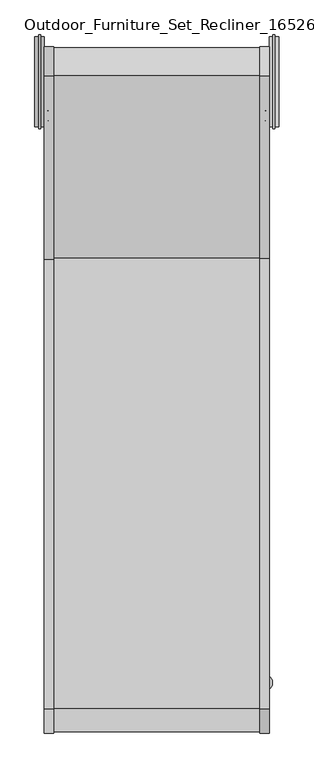
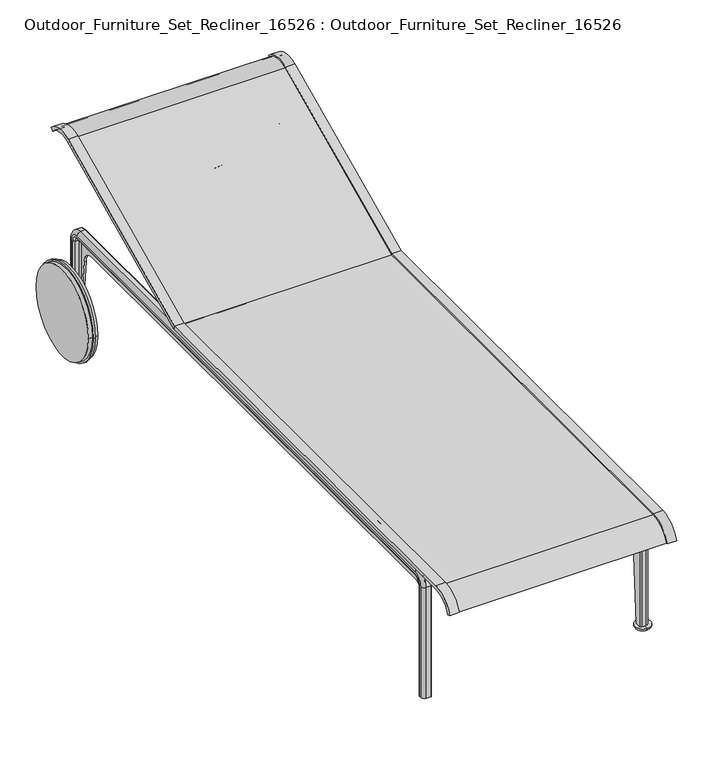
"""IFC4 building model written with IfcOpenShell, lengths in millimetres: furniture geometry, Outdoor_Furniture_Set_Recliner_16526 : Outdoor_Furniture_Set_Recliner_16526."""

from ifc_helpers import new_model, si_unit, point, frame, frame_2d, origin, place, context, project, spatial, polyline, circle_curve, ellipse_curve, trimmed, segment, composite_curve, outline, extrude, source, transform, mapped, element, save
from ifc_brep_helpers import plane_surface, cylinder_surface, revolved_surface, advanced_brep


def outdoor_furniture_set_recliner_16526_outdoor_furniture_set_cea44930(model_context):
    return source(origin(), model_context, "Body", "SolidModel", [
        advanced_brep(
        [(-276.0, -774.0474114, 267.1028811), (-276.0, -739.0647921, 301.0), (-276.0, 739.0647921, 301.0), (-276.0, 774.0474114, 267.1028811), (-276.0, 790.0, 100.0), (-276.0, 807.0, 100.0), (-276.0, 807.0, 320.0), (-276.0, 775.0, 352.0), (-276.0, -775.0, 352.0), (-276.0, -807.0, 320.0), (-276.0, -807.0, 10.0), (-276.0, -790.0, 10.0), (-281.0, 774.0474114, 267.1028811), (-281.0, 739.0647921, 301.0), (-281.0, -739.0647921, 301.0), (-281.0, -774.0474114, 267.1028811), (-281.0, -785.0, 90.583436), (-281.0, -785.0, 320.0), (-281.0, -775.0, 330.0), (-281.0, 775.0, 330.0), (-281.0, 785.0, 320.0), (-281.0, 785.0, 152.374848), (-286.0, 790.0, 100.0), (-286.0, -790.0, 10.0), (-295.0, 790.0, 100.0), (-300.0, 795.0, 100.0), (-300.0, 800.0, 100.0), (-290.0, 810.0, 100.0), (-279.0, 810.0, 100.0), (-290.0, 810.0, 320.0), (-279.0, 810.0, 320.0), (-295.0, 790.0, 320.0), (-286.0, 790.0, 320.0), (-290.0, 775.0, 355.0), (-279.0, 775.0, 355.0), (-295.0, 775.0, 335.0), (-286.0, 775.0, 335.0), (-290.0, -775.0, 355.0), (-279.0, -775.0, 355.0), (-295.0, -775.0, 335.0), (-286.0, -775.0, 335.0), (-290.0, -810.0, 320.0), (-279.0, -810.0, 320.0), (-295.0, -790.0, 320.0), (-286.0, -790.0, 320.0), (-279.0, -810.0, 10.0), (-290.0, -810.0, 10.0), (-300.0, -800.0, 10.0), (-300.0, -795.0, 10.0), (-295.0, -790.0, 10.0), (-300.0, 795.0, 320.0), (-300.0, 775.0, 340.0), (-300.0, -775.0, 340.0), (-300.0, -795.0, 320.0), (-300.0, -800.0, 320.0), (-300.0, -775.0, 345.0), (-300.0, 775.0, 345.0), (-300.0, 800.0, 320.0)],
        [
            (0, 1, circle_curve(frame((-276.0, -739.0647921, 266.0), z_axis=(-1.0, 0.0, 0.0), x_axis=(0.0, 1.0, 0.0)), 35.0)),
            (1, 2),
            (2, 3, circle_curve(frame((-276.0, 739.0647921, 266.0), z_axis=(-1.0, 0.0, 0.0), x_axis=(0.0, 1.0, 0.0)), 35.0)),
            (3, 4),
            (4, 5),
            (5, 6),
            (6, 7, circle_curve(frame((-276.0, 775.0, 320.0), z_axis=(1.0, 0.0, 0.0), x_axis=(0.0, 1.0, 0.0)), 32.0)),
            (7, 8),
            (8, 9, circle_curve(frame((-276.0, -775.0, 320.0), z_axis=(1.0, 0.0, 0.0), x_axis=(0.0, 0.0, 1.0)), 32.0)),
            (9, 10),
            (10, 11),
            (11, 0),
            (12, 13, circle_curve(frame((-281.0, 739.0647921, 266.0), z_axis=(1.0, 0.0, 0.0), x_axis=(0.0, 1.0, 0.0)), 35.0)),
            (13, 14),
            (14, 15, circle_curve(frame((-281.0, -739.0647921, 266.0), z_axis=(1.0, 0.0, 0.0), x_axis=(0.0, 1.0, 0.0)), 35.0)),
            (15, 16),
            (16, 17),
            (17, 18, circle_curve(frame((-281.0, -775.0, 320.0), z_axis=(-1.0, 0.0, 0.0), x_axis=(0.0, 0.0, 1.0)), 10.0)),
            (18, 19),
            (19, 20, circle_curve(frame((-281.0, 775.0, 320.0), z_axis=(-1.0, 0.0, 0.0), x_axis=(0.0, 1.0, 0.0)), 10.0)),
            (20, 21),
            (21, 12),
            (3, 12),
            (21, 22, ellipse_curve(frame((-286.0, 785.0, 152.374848), z_axis=(0.0, 0.9954740654443857, 0.0950335994668569), x_axis=(0.0, -0.09503359946685688, 0.9954740654443857)), 52.6129709, 5.0)),
            (22, 4),
            (15, 0),
            (11, 23),
            (23, 16, ellipse_curve(frame((-286.0, -785.0, 90.583436), z_axis=(0.0, -0.9980805947948747, 0.06192839650684775), x_axis=(0.0, -0.061928396506847755, -0.9980805947948745)), 80.7384057, 5.0)),
            (14, 1),
            (13, 2),
            (24, 25, circle_curve(frame((-295.0, 795.0, 100.0), z_axis=(0.0, 0.0, -1.0), x_axis=(0.0, -1.0, 0.0)), 5.0)),
            (25, 26),
            (26, 27, circle_curve(frame((-290.0, 800.0, 100.0), z_axis=(0.0, 0.0, -1.0), x_axis=(0.0, -1.0, 0.0)), 10.0)),
            (27, 28),
            (28, 5, circle_curve(frame((-279.0, 807.0, 100.0), z_axis=(0.0, 0.0, -1.0), x_axis=(0.0, -1.0, 0.0)), 3.0)),
            (22, 24),
            (27, 29),
            (29, 30),
            (30, 28),
            (30, 6, circle_curve(frame((-279.0, 807.0, 320.0), z_axis=(0.0, 0.0, -1.0), x_axis=(0.0, -1.0, 0.0)), 3.0)),
            (31, 24),
            (22, 32),
            (32, 31),
            (29, 33, circle_curve(frame((-290.0, 775.0, 320.0), z_axis=(1.0, 0.0, 0.0), x_axis=(0.0, 1.0, 0.0)), 35.0)),
            (33, 34),
            (34, 30, circle_curve(frame((-279.0, 775.0, 320.0), z_axis=(-1.0, 0.0, 0.0), x_axis=(0.0, 1.0, 0.0)), 35.0)),
            (34, 7, circle_curve(frame((-279.0, 775.0, 352.0), z_axis=(0.0, 1.0, 0.0), x_axis=(0.0, 0.0, -1.0)), 3.0)),
            (35, 31, circle_curve(frame((-295.0, 775.0, 320.0), z_axis=(-1.0, 0.0, 0.0), x_axis=(0.0, 1.0, 0.0)), 15.0)),
            (32, 36, circle_curve(frame((-286.0, 775.0, 320.0), z_axis=(1.0, 0.0, 0.0), x_axis=(0.0, 1.0, 0.0)), 15.0)),
            (36, 35),
            (33, 37),
            (37, 38),
            (38, 34),
            (38, 8, circle_curve(frame((-279.0, -775.0, 352.0), z_axis=(0.0, 1.0, 0.0), x_axis=(0.0, 0.0, -1.0)), 3.0)),
            (39, 35),
            (36, 40),
            (40, 39),
            (37, 41, circle_curve(frame((-290.0, -775.0, 320.0), z_axis=(1.0, 0.0, 0.0), x_axis=(0.0, 0.0, 1.0)), 35.0)),
            (41, 42),
            (42, 38, circle_curve(frame((-279.0, -775.0, 320.0), z_axis=(-1.0, 0.0, 0.0), x_axis=(0.0, 0.0, 1.0)), 35.0)),
            (42, 9, circle_curve(frame((-279.0, -807.0, 320.0), z_axis=(0.0, 0.0, 1.0), x_axis=(0.0, 1.0, 0.0)), 3.0)),
            (43, 39, circle_curve(frame((-295.0, -775.0, 320.0), z_axis=(-1.0, 0.0, 0.0), x_axis=(0.0, 0.0, 1.0)), 15.0)),
            (40, 44, circle_curve(frame((-286.0, -775.0, 320.0), z_axis=(1.0, 0.0, 0.0), x_axis=(0.0, 0.0, 1.0)), 15.0)),
            (44, 43),
            (10, 45, circle_curve(frame((-279.0, -807.0, 10.0), z_axis=(0.0, 0.0, -1.0), x_axis=(0.0, 1.0, 0.0)), 3.0)),
            (45, 46),
            (46, 47, circle_curve(frame((-290.0, -800.0, 10.0), z_axis=(0.0, 0.0, -1.0), x_axis=(0.0, 1.0, 0.0)), 10.0)),
            (47, 48),
            (48, 49, circle_curve(frame((-295.0, -795.0, 10.0), z_axis=(0.0, 0.0, -1.0), x_axis=(0.0, 1.0, 0.0)), 5.0)),
            (49, 23),
            (41, 46),
            (45, 42),
            (49, 43),
            (44, 23),
            (31, 50, circle_curve(frame((-295.0, 795.0, 320.0), z_axis=(0.0, 0.0, -1.0), x_axis=(0.0, -1.0, 0.0)), 5.0)),
            (50, 25),
            (50, 51, circle_curve(frame((-300.0, 775.0, 320.0), z_axis=(1.0, 0.0, 0.0), x_axis=(0.0, 1.0, 0.0)), 20.0)),
            (51, 52),
            (52, 53, circle_curve(frame((-300.0, -775.0, 320.0), z_axis=(1.0, 0.0, 0.0), x_axis=(0.0, 0.0, 1.0)), 20.0)),
            (53, 48),
            (47, 54),
            (54, 55, circle_curve(frame((-300.0, -775.0, 320.0), z_axis=(-1.0, 0.0, 0.0), x_axis=(0.0, 0.0, 1.0)), 25.0)),
            (55, 56),
            (56, 57, circle_curve(frame((-300.0, 775.0, 320.0), z_axis=(-1.0, 0.0, 0.0), x_axis=(0.0, 1.0, 0.0)), 25.0)),
            (57, 26),
            (57, 29, circle_curve(frame((-290.0, 800.0, 320.0), z_axis=(0.0, 0.0, -1.0), x_axis=(0.0, -1.0, 0.0)), 10.0)),
            (35, 51, circle_curve(frame((-295.0, 775.0, 340.0), z_axis=(0.0, 1.0, 0.0), x_axis=(0.0, 0.0, -1.0)), 5.0)),
            (56, 33, circle_curve(frame((-290.0, 775.0, 345.0), z_axis=(0.0, 1.0, 0.0), x_axis=(0.0, 0.0, -1.0)), 10.0)),
            (39, 52, circle_curve(frame((-295.0, -775.0, 340.0), z_axis=(0.0, 1.0, 0.0), x_axis=(0.0, 0.0, -1.0)), 5.0)),
            (55, 37, circle_curve(frame((-290.0, -775.0, 345.0), z_axis=(0.0, 1.0, 0.0), x_axis=(0.0, 0.0, -1.0)), 10.0)),
            (43, 53, circle_curve(frame((-295.0, -795.0, 320.0), z_axis=(0.0, 0.0, 1.0), x_axis=(0.0, 1.0, 0.0)), 5.0)),
            (54, 41, circle_curve(frame((-290.0, -800.0, 320.0), z_axis=(0.0, 0.0, 1.0), x_axis=(0.0, 1.0, 0.0)), 10.0)),
            (20, 32, circle_curve(frame((-286.0, 785.0, 320.0), z_axis=(0.0, 0.0, 1.0), x_axis=(0.0, -1.0, 0.0)), 5.0)),
            (19, 36, circle_curve(frame((-286.0, 775.0, 330.0), z_axis=(0.0, -1.0, 0.0), x_axis=(0.0, 0.0, -1.0)), 5.0)),
            (18, 40, circle_curve(frame((-286.0, -775.0, 330.0), z_axis=(0.0, -1.0, 0.0), x_axis=(0.0, 0.0, -1.0)), 5.0)),
            (17, 44, circle_curve(frame((-286.0, -785.0, 320.0), z_axis=(0.0, 0.0, -1.0), x_axis=(0.0, 1.0, 0.0)), 5.0)),
        ],
        [
            plane_surface(frame((-276.0, 774.0474114, 267.1028811), z_axis=(1.0, 0.0, 0.0), x_axis=(0.0, 0.0950335994668569, -0.9954740654443857))),
            plane_surface(frame((-281.0, 774.0474114, 267.1028811), z_axis=(-1.0, 0.0, 0.0), x_axis=(0.0, -0.0950335994668569, 0.9954740654443857))),
            plane_surface(frame((-276.0, 774.0474114, 267.1028811), z_axis=(0.0, -0.9954740654443857, -0.0950335994668569), x_axis=(-1.0, 0.0, 0.0))),
            plane_surface(frame((-276.0, -790.0, 10.0), z_axis=(0.0, 0.9980805947948747, -0.06192839650684775), x_axis=(-1.0, 0.0, 0.0))),
            revolved_surface(polyline([(-281.0, -704.0647921, 266.0), (-276.0, -704.0647921, 266.0)]), (-281.0, -739.0647921, 266.0), (-1.0, 0.0, 0.0)),
            plane_surface(frame((-276.0, -739.0647921, 301.0), z_axis=(0.0, 0.0, -1.0), x_axis=(-1.0, 0.0, 0.0))),
            revolved_surface(polyline([(-281.0, 774.0647921, 266.0), (-276.0, 774.0647921, 266.0)]), (-281.0, 739.0647921, 266.0), (-1.0, 0.0, 0.0)),
            plane_surface(frame((0.0, 810.0, 100.0), z_axis=(0.0, 0.0, -1.0), x_axis=(1.0, 0.0, 0.0))),
            plane_surface(frame((-290.0, 810.0, 100.0), z_axis=(0.0, 1.0, 0.0), x_axis=(0.0, 0.0, 1.0))),
            cylinder_surface(frame((-279.0, 807.0, 100.0), z_axis=(0.0, 0.0, -1.0), x_axis=(0.0, -1.0, 0.0)), 3.0),
            plane_surface(frame((-276.0, 790.0, 100.0), z_axis=(0.0, -1.0, 0.0), x_axis=(0.0, 0.0, 1.0))),
            cylinder_surface(frame((0.0, 775.0, 320.0), z_axis=(1.0, 0.0, 0.0), x_axis=(0.0, 1.0, 0.0)), 35.0),
            revolved_surface(trimmed(ellipse_curve(frame((-279.0, 807.0, 320.0), z_axis=(0.0, 0.0, -1.0), x_axis=(0.0, -1.0, 0.0)), 3.0, 3.0), [point((-279.0, 810.0, 320.0))], [point((-276.0, 807.0, 320.0))], True, "CARTESIAN"), (0.0, 775.0, 320.0), (1.0, 0.0, 0.0)),
            revolved_surface(polyline([(-286.0, 790.0, 320.0), (-295.0, 790.0, 320.0)]), (0.0, 775.0, 320.0), (1.0, 0.0, 0.0)),
            plane_surface(frame((-290.0, 775.0, 355.0), z_axis=(0.0, 0.0, 1.0), x_axis=(0.0, -1.0, 0.0))),
            cylinder_surface(frame((-279.0, 775.0, 352.0), z_axis=(0.0, 1.0, 0.0), x_axis=(0.0, 0.0, -1.0)), 3.0),
            plane_surface(frame((-276.0, 775.0, 335.0), z_axis=(0.0, 0.0, -1.0), x_axis=(0.0, -1.0, 0.0))),
            cylinder_surface(frame((0.0, -775.0, 320.0), z_axis=(1.0, 0.0, 0.0), x_axis=(0.0, 0.0, 1.0)), 35.0),
            revolved_surface(trimmed(ellipse_curve(frame((-279.0, -775.0, 352.0), z_axis=(0.0, 1.0, 0.0), x_axis=(0.0, 0.0, -1.0)), 3.0, 3.0), [point((-279.0, -775.0, 355.0))], [point((-276.0, -775.0, 352.0))], True, "CARTESIAN"), (0.0, -775.0, 320.0), (1.0, 0.0, 0.0)),
            revolved_surface(polyline([(-286.0, -775.0, 335.0), (-295.0, -775.0, 335.0)]), (0.0, -775.0, 320.0), (1.0, 0.0, 0.0)),
            plane_surface(frame((0.0, -810.0, 10.0), z_axis=(0.0, 0.0, -1.0), x_axis=(1.0, 0.0, 0.0))),
            plane_surface(frame((-290.0, -810.0, 320.0), z_axis=(0.0, -1.0, 0.0), x_axis=(0.0, 0.0, -1.0))),
            cylinder_surface(frame((-279.0, -807.0, 320.0), z_axis=(0.0, 0.0, 1.0), x_axis=(0.0, 1.0, 0.0)), 3.0),
            plane_surface(frame((-276.0, -790.0, 320.0), z_axis=(0.0, 1.0, 0.0), x_axis=(0.0, 0.0, -1.0))),
            cylinder_surface(frame((-295.0, 795.0, 100.0), z_axis=(0.0, 0.0, -1.0), x_axis=(0.0, -1.0, 0.0)), 5.0),
            plane_surface(frame((-300.0, 795.0, 100.0), z_axis=(-1.0, 0.0, 0.0), x_axis=(0.0, 0.0, 1.0))),
            cylinder_surface(frame((-290.0, 800.0, 100.0), z_axis=(0.0, 0.0, -1.0), x_axis=(0.0, -1.0, 0.0)), 10.0),
            revolved_surface(trimmed(ellipse_curve(frame((-295.0, 795.0, 320.0), z_axis=(0.0, 0.0, -1.0), x_axis=(0.0, -1.0, 0.0)), 5.0, 5.0), [point((-295.0, 790.0, 320.0))], [point((-300.0, 795.0, 320.0))], True, "CARTESIAN"), (0.0, 775.0, 320.0), (1.0, 0.0, 0.0)),
            revolved_surface(trimmed(ellipse_curve(frame((-290.0, 800.0, 320.0), z_axis=(0.0, 0.0, -1.0), x_axis=(0.0, -1.0, 0.0)), 10.0, 10.0), [point((-300.0, 800.0, 320.0))], [point((-290.0, 810.0, 320.0))], True, "CARTESIAN"), (0.0, 775.0, 320.0), (1.0, 0.0, 0.0)),
            cylinder_surface(frame((-295.0, 775.0, 340.0), z_axis=(0.0, 1.0, 0.0), x_axis=(0.0, 0.0, -1.0)), 5.0),
            cylinder_surface(frame((-290.0, 775.0, 345.0), z_axis=(0.0, 1.0, 0.0), x_axis=(0.0, 0.0, -1.0)), 10.0),
            revolved_surface(trimmed(ellipse_curve(frame((-295.0, -775.0, 340.0), z_axis=(0.0, 1.0, 0.0), x_axis=(0.0, 0.0, -1.0)), 5.0, 5.0), [point((-295.0, -775.0, 335.0))], [point((-300.0, -775.0, 340.0))], True, "CARTESIAN"), (0.0, -775.0, 320.0), (1.0, 0.0, 0.0)),
            revolved_surface(trimmed(ellipse_curve(frame((-290.0, -775.0, 345.0), z_axis=(0.0, 1.0, 0.0), x_axis=(0.0, 0.0, -1.0)), 10.0, 10.0), [point((-300.0, -775.0, 345.0))], [point((-290.0, -775.0, 355.0))], True, "CARTESIAN"), (0.0, -775.0, 320.0), (1.0, 0.0, 0.0)),
            cylinder_surface(frame((-295.0, -795.0, 320.0), z_axis=(0.0, 0.0, 1.0), x_axis=(0.0, 1.0, 0.0)), 5.0),
            cylinder_surface(frame((-290.0, -800.0, 320.0), z_axis=(0.0, 0.0, 1.0), x_axis=(0.0, 1.0, 0.0)), 10.0),
            revolved_surface(polyline([(-286.0, 780.0, 320.0), (-286.0, 780.0, 99.99999996306983)]), (-286.0, 785.0, 100.0), (0.0, 0.0, 1.0)),
            revolved_surface(trimmed(ellipse_curve(frame((-286.0, 785.0, 320.0), z_axis=(0.0, 0.0, 1.0), x_axis=(0.0, -1.0, 0.0)), 5.0, 5.0), [point((-281.0, 785.0, 320.0))], [point((-286.0, 790.0, 320.0))], True, "CARTESIAN"), (0.0, 775.0, 320.0), (1.0, 0.0, 0.0)),
            revolved_surface(polyline([(-286.0, -775.0, 325.0), (-286.0, 775.0, 325.0)]), (-286.0, 775.0, 330.0), (0.0, -1.0, 0.0)),
            revolved_surface(trimmed(ellipse_curve(frame((-286.0, -775.0, 330.0), z_axis=(0.0, -1.0, 0.0), x_axis=(0.0, 0.0, -1.0)), 5.0, 5.0), [point((-281.0, -775.0, 330.0))], [point((-286.0, -775.0, 335.0))], True, "CARTESIAN"), (0.0, -775.0, 320.0), (1.0, 0.0, 0.0)),
            revolved_surface(polyline([(-286.0, -780.0, 10.0), (-286.0, -780.0, 320.0)]), (-286.0, -785.0, 320.0), (0.0, 0.0, -1.0)),
        ],
        [
            (0, [[1, 2, 3, 4, 5, 6, 7, 8, 9, 10, 11, 12]]),
            (1, [[13, 14, 15, 16, 17, 18, 19, 20, 21, 22]]),
            (2, [[23, -22, 24, 25, -4]]),
            (3, [[26, -12, 27, 28, -16]]),
            (4, [[-1, -26, -15, 29]]),
            (5, [[-2, -29, -14, 30]]),
            (6, [[-3, -30, -13, -23]]),
            (7, [[31, 32, 33, 34, 35, -5, -25, 36]]),
            (8, [[-34, 37, 38, 39]]),
            (9, [[-35, -39, 40, -6]]),
            (10, [[41, -36, 42, 43]]),
            (11, [[-38, 44, 45, 46]]),
            (12, [[-40, -46, 47, -7]]),
            (13, [[48, -43, 49, 50]]),
            (14, [[-45, 51, 52, 53]]),
            (15, [[-8, -47, -53, 54]]),
            (16, [[55, -50, 56, 57]]),
            (17, [[-52, 58, 59, 60]]),
            (18, [[-9, -54, -60, 61]]),
            (19, [[62, -57, 63, 64]]),
            (20, [[-11, 65, 66, 67, 68, 69, 70, -27]]),
            (21, [[-59, 71, -66, 72]]),
            (22, [[-10, -61, -72, -65]]),
            (23, [[73, -64, 74, -70]]),
            (24, [[-31, -41, 75, 76]]),
            (25, [[-32, -76, 77, 78, 79, 80, -68, 81, 82, 83, 84, 85]]),
            (26, [[-33, -85, 86, -37]]),
            (27, [[-48, 87, -77, -75]]),
            (28, [[-44, -86, -84, 88]]),
            (29, [[-55, 89, -78, -87]]),
            (30, [[-51, -88, -83, 90]]),
            (31, [[-62, 91, -79, -89]]),
            (32, [[-58, -90, -82, 92]]),
            (33, [[-69, -80, -91, -73]]),
            (34, [[-67, -71, -92, -81]]),
            (35, [[93, -42, -24, -21]]),
            (36, [[-93, -20, 94, -49]]),
            (37, [[-94, -19, 95, -56]]),
            (38, [[-95, -18, 96, -63]]),
            (39, [[-96, -17, -28, -74]]),
        ],
    ),
        advanced_brep(
        [(286.0, 790.0, 100.0), (281.0, 785.0, 152.374848), (281.0, 774.0474114, 267.1028811), (276.0, 774.0474114, 267.1028811), (276.0, 790.0, 100.0), (276.0, -790.0, 10.0), (276.0, -774.0474114, 267.1028811), (281.0, -774.0474114, 267.1028811), (281.0, -785.0, 90.583436), (286.0, -790.0, 10.0), (276.0, 807.0, 100.0), (279.0, 810.0, 100.0), (290.0, 810.0, 100.0), (300.0, 800.0, 100.0), (300.0, 795.0, 100.0), (295.0, 790.0, 100.0), (295.0, -790.0, 10.0), (300.0, -795.0, 10.0), (300.0, -800.0, 10.0), (290.0, -810.0, 10.0), (279.0, -810.0, 10.0), (276.0, -807.0, 10.0), (295.0, 790.0, 320.0), (286.0, 790.0, 320.0), (276.0, 739.0647921, 301.0), (276.0, -739.0647921, 301.0), (276.0, -807.0, 320.0), (276.0, -775.0, 352.0), (276.0, 775.0, 352.0), (276.0, 807.0, 320.0), (279.0, 810.0, 320.0), (290.0, 810.0, 320.0), (300.0, 800.0, 320.0), (300.0, 775.0, 345.0), (300.0, -775.0, 345.0), (300.0, -800.0, 320.0), (300.0, -795.0, 320.0), (300.0, -775.0, 340.0), (300.0, 775.0, 340.0), (300.0, 795.0, 320.0), (295.0, 775.0, 335.0), (286.0, 775.0, 335.0), (279.0, 775.0, 355.0), (290.0, 775.0, 355.0), (295.0, -775.0, 335.0), (286.0, -775.0, 335.0), (279.0, -775.0, 355.0), (290.0, -775.0, 355.0), (295.0, -790.0, 320.0), (286.0, -790.0, 320.0), (279.0, -810.0, 320.0), (290.0, -810.0, 320.0), (281.0, -739.0647921, 301.0), (281.0, 739.0647921, 301.0), (281.0, 785.0, 320.0), (281.0, 775.0, 330.0), (281.0, -775.0, 330.0), (281.0, -785.0, 320.0)],
        [
            (0, 1, ellipse_curve(frame((286.0, 785.0, 152.374848), z_axis=(0.0, 0.9954740654443857, 0.0950335994668569), x_axis=(0.0, -0.09503359946685688, 0.9954740654443857)), 52.6129709, 5.0)),
            (1, 2),
            (2, 3),
            (3, 4),
            (4, 0),
            (5, 6),
            (6, 7),
            (7, 8),
            (8, 9, ellipse_curve(frame((286.0, -785.0, 90.583436), z_axis=(0.0, -0.9980805947948747, 0.06192839650684775), x_axis=(0.0, -0.061928396506847755, -0.9980805947948745)), 80.7384057, 5.0)),
            (9, 5),
            (4, 10),
            (10, 11, circle_curve(frame((279.0, 807.0, 100.0), z_axis=(0.0, 0.0, -1.0), x_axis=(0.0, -1.0, 0.0)), 3.0)),
            (11, 12),
            (12, 13, circle_curve(frame((290.0, 800.0, 100.0), z_axis=(0.0, 0.0, -1.0), x_axis=(0.0, -1.0, 0.0)), 10.0)),
            (13, 14),
            (14, 15, circle_curve(frame((295.0, 795.0, 100.0), z_axis=(0.0, 0.0, -1.0), x_axis=(0.0, -1.0, 0.0)), 5.0)),
            (15, 0),
            (16, 17, circle_curve(frame((295.0, -795.0, 10.0), z_axis=(0.0, 0.0, -1.0), x_axis=(0.0, 1.0, 0.0)), 5.0)),
            (17, 18),
            (18, 19, circle_curve(frame((290.0, -800.0, 10.0), z_axis=(0.0, 0.0, -1.0), x_axis=(0.0, 1.0, 0.0)), 10.0)),
            (19, 20),
            (20, 21, circle_curve(frame((279.0, -807.0, 10.0), z_axis=(0.0, 0.0, -1.0), x_axis=(0.0, 1.0, 0.0)), 3.0)),
            (21, 5),
            (9, 16),
            (15, 22),
            (22, 23),
            (23, 0),
            (3, 24, circle_curve(frame((276.0, 739.0647921, 266.0), z_axis=(1.0, 0.0, 0.0), x_axis=(0.0, 1.0, 0.0)), 35.0)),
            (24, 25),
            (25, 6, circle_curve(frame((276.0, -739.0647921, 266.0), z_axis=(1.0, 0.0, 0.0), x_axis=(0.0, 1.0, 0.0)), 35.0)),
            (21, 26),
            (26, 27, circle_curve(frame((276.0, -775.0, 320.0), z_axis=(-1.0, 0.0, 0.0), x_axis=(0.0, 0.0, 1.0)), 32.0)),
            (27, 28),
            (28, 29, circle_curve(frame((276.0, 775.0, 320.0), z_axis=(-1.0, 0.0, 0.0), x_axis=(0.0, 1.0, 0.0)), 32.0)),
            (29, 10),
            (29, 30, circle_curve(frame((279.0, 807.0, 320.0), z_axis=(0.0, 0.0, -1.0), x_axis=(0.0, -1.0, 0.0)), 3.0)),
            (30, 11),
            (30, 31),
            (31, 12),
            (31, 32, circle_curve(frame((290.0, 800.0, 320.0), z_axis=(0.0, 0.0, -1.0), x_axis=(0.0, -1.0, 0.0)), 10.0)),
            (32, 13),
            (32, 33, circle_curve(frame((300.0, 775.0, 320.0), z_axis=(1.0, 0.0, 0.0), x_axis=(0.0, 1.0, 0.0)), 25.0)),
            (33, 34),
            (34, 35, circle_curve(frame((300.0, -775.0, 320.0), z_axis=(1.0, 0.0, 0.0), x_axis=(0.0, 0.0, 1.0)), 25.0)),
            (35, 18),
            (17, 36),
            (36, 37, circle_curve(frame((300.0, -775.0, 320.0), z_axis=(-1.0, 0.0, 0.0), x_axis=(0.0, 0.0, 1.0)), 20.0)),
            (37, 38),
            (38, 39, circle_curve(frame((300.0, 775.0, 320.0), z_axis=(-1.0, 0.0, 0.0), x_axis=(0.0, 1.0, 0.0)), 20.0)),
            (39, 14),
            (39, 22, circle_curve(frame((295.0, 795.0, 320.0), z_axis=(0.0, 0.0, -1.0), x_axis=(0.0, -1.0, 0.0)), 5.0)),
            (22, 40, circle_curve(frame((295.0, 775.0, 320.0), z_axis=(1.0, 0.0, 0.0), x_axis=(0.0, 1.0, 0.0)), 15.0)),
            (40, 41),
            (41, 23, circle_curve(frame((286.0, 775.0, 320.0), z_axis=(-1.0, 0.0, 0.0), x_axis=(0.0, 1.0, 0.0)), 15.0)),
            (28, 42, circle_curve(frame((279.0, 775.0, 352.0), z_axis=(0.0, 1.0, 0.0), x_axis=(0.0, 0.0, -1.0)), 3.0)),
            (42, 30, circle_curve(frame((279.0, 775.0, 320.0), z_axis=(-1.0, 0.0, 0.0), x_axis=(0.0, 1.0, 0.0)), 35.0)),
            (42, 43),
            (43, 31, circle_curve(frame((290.0, 775.0, 320.0), z_axis=(-1.0, 0.0, 0.0), x_axis=(0.0, 1.0, 0.0)), 35.0)),
            (43, 33, circle_curve(frame((290.0, 775.0, 345.0), z_axis=(0.0, 1.0, 0.0), x_axis=(0.0, 0.0, -1.0)), 10.0)),
            (38, 40, circle_curve(frame((295.0, 775.0, 340.0), z_axis=(0.0, 1.0, 0.0), x_axis=(0.0, 0.0, -1.0)), 5.0)),
            (40, 44),
            (44, 45),
            (45, 41),
            (27, 46, circle_curve(frame((279.0, -775.0, 352.0), z_axis=(0.0, 1.0, 0.0), x_axis=(0.0, 0.0, -1.0)), 3.0)),
            (46, 42),
            (46, 47),
            (47, 43),
            (47, 34, circle_curve(frame((290.0, -775.0, 345.0), z_axis=(0.0, 1.0, 0.0), x_axis=(0.0, 0.0, -1.0)), 10.0)),
            (37, 44, circle_curve(frame((295.0, -775.0, 340.0), z_axis=(0.0, 1.0, 0.0), x_axis=(0.0, 0.0, -1.0)), 5.0)),
            (44, 48, circle_curve(frame((295.0, -775.0, 320.0), z_axis=(1.0, 0.0, 0.0), x_axis=(0.0, 0.0, 1.0)), 15.0)),
            (48, 49),
            (49, 45, circle_curve(frame((286.0, -775.0, 320.0), z_axis=(-1.0, 0.0, 0.0), x_axis=(0.0, 0.0, 1.0)), 15.0)),
            (26, 50, circle_curve(frame((279.0, -807.0, 320.0), z_axis=(0.0, 0.0, 1.0), x_axis=(0.0, 1.0, 0.0)), 3.0)),
            (50, 46, circle_curve(frame((279.0, -775.0, 320.0), z_axis=(-1.0, 0.0, 0.0), x_axis=(0.0, 0.0, 1.0)), 35.0)),
            (50, 51),
            (51, 47, circle_curve(frame((290.0, -775.0, 320.0), z_axis=(-1.0, 0.0, 0.0), x_axis=(0.0, 0.0, 1.0)), 35.0)),
            (51, 35, circle_curve(frame((290.0, -800.0, 320.0), z_axis=(0.0, 0.0, 1.0), x_axis=(0.0, 1.0, 0.0)), 10.0)),
            (36, 48, circle_curve(frame((295.0, -795.0, 320.0), z_axis=(0.0, 0.0, 1.0), x_axis=(0.0, 1.0, 0.0)), 5.0)),
            (48, 16),
            (9, 49),
            (20, 50),
            (19, 51),
            (7, 52, circle_curve(frame((281.0, -739.0647921, 266.0), z_axis=(-1.0, 0.0, 0.0), x_axis=(0.0, 1.0, 0.0)), 35.0)),
            (52, 53),
            (53, 2, circle_curve(frame((281.0, 739.0647921, 266.0), z_axis=(-1.0, 0.0, 0.0), x_axis=(0.0, 1.0, 0.0)), 35.0)),
            (1, 54),
            (54, 55, circle_curve(frame((281.0, 775.0, 320.0), z_axis=(1.0, 0.0, 0.0), x_axis=(0.0, 1.0, 0.0)), 10.0)),
            (55, 56),
            (56, 57, circle_curve(frame((281.0, -775.0, 320.0), z_axis=(1.0, 0.0, 0.0), x_axis=(0.0, 0.0, 1.0)), 10.0)),
            (57, 8),
            (25, 52),
            (24, 53),
            (23, 54, circle_curve(frame((286.0, 785.0, 320.0), z_axis=(0.0, 0.0, 1.0), x_axis=(0.0, -1.0, 0.0)), 5.0)),
            (41, 55, circle_curve(frame((286.0, 775.0, 330.0), z_axis=(0.0, -1.0, 0.0), x_axis=(0.0, 0.0, -1.0)), 5.0)),
            (45, 56, circle_curve(frame((286.0, -775.0, 330.0), z_axis=(0.0, -1.0, 0.0), x_axis=(0.0, 0.0, -1.0)), 5.0)),
            (49, 57, circle_curve(frame((286.0, -785.0, 320.0), z_axis=(0.0, 0.0, -1.0), x_axis=(0.0, 1.0, 0.0)), 5.0)),
        ],
        [
            plane_surface(frame((-276.0, 774.0474114, 267.1028811), z_axis=(0.0, -0.9954740654443857, -0.0950335994668569), x_axis=(-1.0, 0.0, 0.0))),
            plane_surface(frame((-276.0, -790.0, 10.0), z_axis=(0.0, 0.9980805947948747, -0.06192839650684775), x_axis=(-1.0, 0.0, 0.0))),
            plane_surface(frame((0.0, 810.0, 100.0), z_axis=(0.0, 0.0, -1.0), x_axis=(1.0, 0.0, 0.0))),
            plane_surface(frame((0.0, -810.0, 10.0), z_axis=(0.0, 0.0, -1.0), x_axis=(1.0, 0.0, 0.0))),
            plane_surface(frame((295.0, 790.0, 100.0), z_axis=(0.0, -1.0, 0.0), x_axis=(0.0, 0.0, 1.0))),
            plane_surface(frame((276.0, 790.0, 100.0), z_axis=(-1.0, 0.0, 0.0), x_axis=(0.0, 0.0, 1.0))),
            cylinder_surface(frame((279.0, 807.0, 100.0), z_axis=(0.0, 0.0, -1.0), x_axis=(0.0, -1.0, 0.0)), 3.0),
            plane_surface(frame((279.0, 810.0, 100.0), z_axis=(0.0, 1.0, 0.0), x_axis=(0.0, 0.0, 1.0))),
            cylinder_surface(frame((290.0, 800.0, 100.0), z_axis=(0.0, 0.0, -1.0), x_axis=(0.0, -1.0, 0.0)), 10.0),
            plane_surface(frame((300.0, 800.0, 100.0), z_axis=(1.0, 0.0, 0.0), x_axis=(0.0, 0.0, 1.0))),
            cylinder_surface(frame((295.0, 795.0, 100.0), z_axis=(0.0, 0.0, -1.0), x_axis=(0.0, -1.0, 0.0)), 5.0),
            revolved_surface(polyline([(295.0, 790.0, 320.0), (286.0, 790.0, 320.0)]), (0.0, 775.0, 320.0), (1.0, 0.0, 0.0)),
            revolved_surface(trimmed(ellipse_curve(frame((279.0, 807.0, 320.0), z_axis=(0.0, 0.0, -1.0), x_axis=(0.0, -1.0, 0.0)), 3.0, 3.0), [point((276.0, 807.0, 320.0))], [point((279.0, 810.0, 320.0))], True, "CARTESIAN"), (0.0, 775.0, 320.0), (1.0, 0.0, 0.0)),
            cylinder_surface(frame((0.0, 775.0, 320.0), z_axis=(1.0, 0.0, 0.0), x_axis=(0.0, 1.0, 0.0)), 35.0),
            revolved_surface(trimmed(ellipse_curve(frame((290.0, 800.0, 320.0), z_axis=(0.0, 0.0, -1.0), x_axis=(0.0, -1.0, 0.0)), 10.0, 10.0), [point((290.0, 810.0, 320.0))], [point((300.0, 800.0, 320.0))], True, "CARTESIAN"), (0.0, 775.0, 320.0), (1.0, 0.0, 0.0)),
            revolved_surface(trimmed(ellipse_curve(frame((295.0, 795.0, 320.0), z_axis=(0.0, 0.0, -1.0), x_axis=(0.0, -1.0, 0.0)), 5.0, 5.0), [point((300.0, 795.0, 320.0))], [point((295.0, 790.0, 320.0))], True, "CARTESIAN"), (0.0, 775.0, 320.0), (1.0, 0.0, 0.0)),
            plane_surface(frame((295.0, 775.0, 335.0), z_axis=(0.0, 0.0, -1.0), x_axis=(0.0, -1.0, 0.0))),
            cylinder_surface(frame((279.0, 775.0, 352.0), z_axis=(0.0, 1.0, 0.0), x_axis=(0.0, 0.0, -1.0)), 3.0),
            plane_surface(frame((279.0, 775.0, 355.0), z_axis=(0.0, 0.0, 1.0), x_axis=(0.0, -1.0, 0.0))),
            cylinder_surface(frame((290.0, 775.0, 345.0), z_axis=(0.0, 1.0, 0.0), x_axis=(0.0, 0.0, -1.0)), 10.0),
            cylinder_surface(frame((295.0, 775.0, 340.0), z_axis=(0.0, 1.0, 0.0), x_axis=(0.0, 0.0, -1.0)), 5.0),
            revolved_surface(polyline([(295.0, -775.0, 335.0), (286.0, -775.0, 335.0)]), (0.0, -775.0, 320.0), (1.0, 0.0, 0.0)),
            revolved_surface(trimmed(ellipse_curve(frame((279.0, -775.0, 352.0), z_axis=(0.0, 1.0, 0.0), x_axis=(0.0, 0.0, -1.0)), 3.0, 3.0), [point((276.0, -775.0, 352.0))], [point((279.0, -775.0, 355.0))], True, "CARTESIAN"), (0.0, -775.0, 320.0), (1.0, 0.0, 0.0)),
            cylinder_surface(frame((0.0, -775.0, 320.0), z_axis=(1.0, 0.0, 0.0), x_axis=(0.0, 0.0, 1.0)), 35.0),
            revolved_surface(trimmed(ellipse_curve(frame((290.0, -775.0, 345.0), z_axis=(0.0, 1.0, 0.0), x_axis=(0.0, 0.0, -1.0)), 10.0, 10.0), [point((290.0, -775.0, 355.0))], [point((300.0, -775.0, 345.0))], True, "CARTESIAN"), (0.0, -775.0, 320.0), (1.0, 0.0, 0.0)),
            revolved_surface(trimmed(ellipse_curve(frame((295.0, -775.0, 340.0), z_axis=(0.0, 1.0, 0.0), x_axis=(0.0, 0.0, -1.0)), 5.0, 5.0), [point((300.0, -775.0, 340.0))], [point((295.0, -775.0, 335.0))], True, "CARTESIAN"), (0.0, -775.0, 320.0), (1.0, 0.0, 0.0)),
            plane_surface(frame((295.0, -790.0, 320.0), z_axis=(0.0, 1.0, 0.0), x_axis=(0.0, 0.0, -1.0))),
            cylinder_surface(frame((279.0, -807.0, 320.0), z_axis=(0.0, 0.0, 1.0), x_axis=(0.0, 1.0, 0.0)), 3.0),
            plane_surface(frame((279.0, -810.0, 320.0), z_axis=(0.0, -1.0, 0.0), x_axis=(0.0, 0.0, -1.0))),
            cylinder_surface(frame((290.0, -800.0, 320.0), z_axis=(0.0, 0.0, 1.0), x_axis=(0.0, 1.0, 0.0)), 10.0),
            cylinder_surface(frame((295.0, -795.0, 320.0), z_axis=(0.0, 0.0, 1.0), x_axis=(0.0, 1.0, 0.0)), 5.0),
            plane_surface(frame((281.0, 774.0647921, 266.0), z_axis=(1.0, 0.0, 0.0), x_axis=(0.0, 0.0, -1.0))),
            revolved_surface(polyline([(281.0, -704.0647921, 266.0), (276.0, -704.0647921, 266.0)]), (281.0, -739.0647921, 266.0), (1.0, 0.0, 0.0)),
            plane_surface(frame((276.0, 739.0647921, 301.0), z_axis=(0.0, 0.0, -1.0), x_axis=(1.0, 0.0, 0.0))),
            revolved_surface(polyline([(281.0, 774.0647921, 266.0), (276.0, 774.0647921, 266.0)]), (281.0, 739.0647921, 266.0), (1.0, 0.0, 0.0)),
            revolved_surface(polyline([(286.0, 780.0, 320.0), (286.0, 780.0, 99.99999996306983)]), (286.0, 785.0, 100.0), (0.0, 0.0, 1.0)),
            revolved_surface(trimmed(ellipse_curve(frame((286.0, 785.0, 320.0), z_axis=(0.0, 0.0, 1.0), x_axis=(0.0, -1.0, 0.0)), 5.0, 5.0), [point((286.0, 790.0, 320.0))], [point((281.0, 785.0, 320.0))], True, "CARTESIAN"), (0.0, 775.0, 320.0), (1.0, 0.0, 0.0)),
            revolved_surface(polyline([(286.0, -775.0, 325.0), (286.0, 775.0, 325.0)]), (286.0, 775.0, 330.0), (0.0, -1.0, 0.0)),
            revolved_surface(trimmed(ellipse_curve(frame((286.0, -775.0, 330.0), z_axis=(0.0, -1.0, 0.0), x_axis=(0.0, 0.0, -1.0)), 5.0, 5.0), [point((286.0, -775.0, 335.0))], [point((281.0, -775.0, 330.0))], True, "CARTESIAN"), (0.0, -775.0, 320.0), (1.0, 0.0, 0.0)),
            revolved_surface(polyline([(286.0, -780.0, 10.0), (286.0, -780.0, 320.0)]), (286.0, -785.0, 320.0), (0.0, 0.0, -1.0)),
        ],
        [
            (0, [[1, 2, 3, 4, 5]]),
            (1, [[6, 7, 8, 9, 10]]),
            (2, [[-5, 11, 12, 13, 14, 15, 16, 17]]),
            (3, [[18, 19, 20, 21, 22, 23, -10, 24]]),
            (4, [[25, 26, 27, -17]]),
            (5, [[-11, -4, 28, 29, 30, -6, -23, 31, 32, 33, 34, 35]]),
            (6, [[-12, -35, 36, 37]]),
            (7, [[-13, -37, 38, 39]]),
            (8, [[-14, -39, 40, 41]]),
            (9, [[-15, -41, 42, 43, 44, 45, -19, 46, 47, 48, 49, 50]]),
            (10, [[-16, -50, 51, -25]]),
            (11, [[52, 53, 54, -26]]),
            (12, [[-34, 55, 56, -36]]),
            (13, [[-38, -56, 57, 58]]),
            (14, [[-40, -58, 59, -42]]),
            (15, [[-49, 60, -52, -51]]),
            (16, [[61, 62, 63, -53]]),
            (17, [[-33, 64, 65, -55]]),
            (18, [[-57, -65, 66, 67]]),
            (19, [[-43, -59, -67, 68]]),
            (20, [[-48, 69, -61, -60]]),
            (21, [[70, 71, 72, -62]]),
            (22, [[-32, 73, 74, -64]]),
            (23, [[-66, -74, 75, 76]]),
            (24, [[-44, -68, -76, 77]]),
            (25, [[-47, 78, -70, -69]]),
            (26, [[79, -24, 80, -71]]),
            (27, [[-22, 81, -73, -31]]),
            (28, [[-21, 82, -75, -81]]),
            (29, [[-20, -45, -77, -82]]),
            (30, [[-18, -79, -78, -46]]),
            (31, [[83, 84, 85, -2, 86, 87, 88, 89, 90, -8]]),
            (32, [[-30, 91, -83, -7]]),
            (33, [[-29, 92, -84, -91]]),
            (34, [[-28, -3, -85, -92]]),
            (35, [[93, -86, -1, -27]]),
            (36, [[-93, -54, 94, -87]]),
            (37, [[-94, -63, 95, -88]]),
            (38, [[-95, -72, 96, -89]]),
            (39, [[-96, -80, -9, -90]]),
        ],
    ),
        extrude(outline(composite_curve([segment(polyline([(-870.0, 361.0), (330.0, 361.0), (330.0, 359.0), (-870.0, 359.0)]), True, "CONTINUOUS"), segment(trimmed(circle_curve(frame_2d((-870.0, 296.4702225)), 62.5297775), [point((-870.0, 359.0))], [point((-928.7587705, 317.856666))], True, "CARTESIAN"), True, "CONTINUOUS"), segment(polyline([(-928.7587705, 317.856666), (-930.6381557, 318.5407063)]), True, "CONTINUOUS"), segment(trimmed(circle_curve(frame_2d((-870.0, 296.4702225)), 64.5297775), [point((-930.6381557, 318.5407063))], [point((-870.0, 361.0))], False, "CARTESIAN"), True, "CONTINUOUS")], self_intersect=False)), frame((-275.0, 0.0, 0.0), z_axis=(1.0, 0.0, 0.0), x_axis=(0.0, 1.0, 0.0)), (0.0, 0.0, 1.0), 550.0),
        extrude(outline(composite_curve([segment(trimmed(circle_curve(frame_2d((-870.0, 296.4702225)), 58.5297775), [point((-870.0, 355.0))], [point((-925.0, 316.4885854))], True, "CARTESIAN"), True, "CONTINUOUS"), segment(polyline([(-925.0, 316.4885854), (-934.3969262, 319.9087868)]), True, "CONTINUOUS"), segment(trimmed(circle_curve(frame_2d((-870.0, 296.4702225)), 68.5297775), [point((-934.3969262, 319.9087868))], [point((-870.0, 365.0))], False, "CARTESIAN"), True, "CONTINUOUS"), segment(polyline([(-870.0, 365.0), (330.0, 365.0), (330.0, 355.0), (-870.0, 355.0)]), True, "CONTINUOUS")], self_intersect=False)), frame((275.0, 0.0, 0.0), z_axis=(1.0, 0.0, 0.0), x_axis=(0.0, 1.0, 0.0)), (0.0, 0.0, 1.0), 25.0),
        extrude(outline(composite_curve([segment(polyline([(327.4642904, 360.4378467), (816.8704954, 588.6517081)]), True, "CONTINUOUS"), segment(trimmed(circle_curve(frame_2d((844.1419578, 530.1678682)), 64.5297775), [point((816.8704954, 588.6517081))], [point((889.7714011, 575.7973115))], False, "CARTESIAN"), True, "CONTINUOUS"), segment(polyline([(889.7714011, 575.7973115), (888.3571875, 574.3830979)]), True, "CONTINUOUS"), segment(trimmed(circle_curve(frame_2d((844.1419578, 530.1678682)), 62.5297775), [point((888.3571875, 574.3830979))], [point((817.715732, 586.8390925))], True, "CARTESIAN"), True, "CONTINUOUS"), segment(polyline([(817.715732, 586.8390925), (328.309527, 358.6252311), (327.4642904, 360.4378467)]), True, "CONTINUOUS")], self_intersect=False)), frame((-275.0, 0.0, 0.0), z_axis=(1.0, 0.0, 0.0), x_axis=(0.0, 1.0, 0.0)), (0.0, 0.0, 1.0), 550.0),
        extrude(outline(composite_curve([segment(polyline([(819.406205, 583.2138613), (330.0, 355.0), (325.7738174, 364.0630779), (815.1800224, 592.2769392)]), True, "CONTINUOUS"), segment(trimmed(circle_curve(frame_2d((844.1419578, 530.1678682)), 68.5297775), [point((815.1800224, 592.2769392))], [point((892.5998282, 578.6257386))], False, "CARTESIAN"), True, "CONTINUOUS"), segment(polyline([(892.5998282, 578.6257386), (885.5287604, 571.5546708)]), True, "CONTINUOUS"), segment(trimmed(circle_curve(frame_2d((844.1419578, 530.1678682)), 58.5297775), [point((885.5287604, 571.5546708))], [point((819.406205, 583.2138613))], True, "CARTESIAN"), True, "CONTINUOUS")], self_intersect=False)), frame((-300.0, 0.0, 0.0), z_axis=(1.0, 0.0, 0.0), x_axis=(0.0, 1.0, 0.0)), (0.0, 0.0, 1.0), 25.0),
        extrude(outline(composite_curve([segment(polyline([(819.406205, 583.2138613), (330.0, 355.0), (325.7738174, 364.0630779), (815.1800224, 592.2769392)]), True, "CONTINUOUS"), segment(trimmed(circle_curve(frame_2d((844.1419578, 530.1678682)), 68.5297775), [point((815.1800224, 592.2769392))], [point((892.5998282, 578.6257386))], False, "CARTESIAN"), True, "CONTINUOUS"), segment(polyline([(892.5998282, 578.6257386), (885.5287604, 571.5546708)]), True, "CONTINUOUS"), segment(trimmed(circle_curve(frame_2d((844.1419578, 530.1678682)), 58.5297775), [point((885.5287604, 571.5546708))], [point((819.406205, 583.2138613))], True, "CARTESIAN"), True, "CONTINUOUS")], self_intersect=False)), frame((275.0, 0.0, 0.0), z_axis=(1.0, 0.0, 0.0), x_axis=(0.0, 1.0, 0.0)), (0.0, 0.0, 1.0), 25.0),
        extrude(outline(composite_curve([segment(trimmed(circle_curve(frame_2d((-870.0, 296.4702225)), 58.5297775), [point((-870.0, 355.0))], [point((-925.0, 316.4885854))], True, "CARTESIAN"), True, "CONTINUOUS"), segment(polyline([(-925.0, 316.4885854), (-934.3969262, 319.9087868)]), True, "CONTINUOUS"), segment(trimmed(circle_curve(frame_2d((-870.0, 296.4702225)), 68.5297775), [point((-934.3969262, 319.9087868))], [point((-870.0, 365.0))], False, "CARTESIAN"), True, "CONTINUOUS"), segment(polyline([(-870.0, 365.0), (330.0, 365.0), (330.0, 355.0), (-870.0, 355.0)]), True, "CONTINUOUS")], self_intersect=False)), frame((-300.0, 0.0, 0.0), z_axis=(1.0, 0.0, 0.0), x_axis=(0.0, 1.0, 0.0)), (0.0, 0.0, 1.0), 25.0),
        extrude(outline(composite_curve([segment(trimmed(circle_curve(frame_2d((799.0, 125.0)), 120.0), [point((919.0, 125.0))], [point((679.0, 125.0))], False, "CARTESIAN"), True, "CONTINUOUS"), segment(trimmed(circle_curve(frame_2d((799.0, 125.0)), 120.0), [point((679.0, 125.0))], [point((919.0, 125.0))], False, "CARTESIAN"), True, "CONTINUOUS")], self_intersect=False)), frame((-325.0, 0.0, 0.0), z_axis=(1.0, 0.0, 0.0), x_axis=(0.0, 1.0, 0.0)), (0.0, 0.0, 1.0), 25.0),
        extrude(outline(composite_curve([segment(trimmed(circle_curve(frame_2d((799.0, 125.0)), 120.0), [point((919.0, 125.0))], [point((679.0, 125.0))], False, "CARTESIAN"), True, "CONTINUOUS"), segment(trimmed(circle_curve(frame_2d((799.0, 125.0)), 120.0), [point((679.0, 125.0))], [point((919.0, 125.0))], False, "CARTESIAN"), True, "CONTINUOUS")], self_intersect=False)), frame((300.0, 0.0, 0.0), z_axis=(1.0, 0.0, 0.0), x_axis=(0.0, 1.0, 0.0)), (0.0, 0.0, 1.0), 25.0),
        extrude(outline(composite_curve([segment(trimmed(circle_curve(frame_2d((799.0, 125.0)), 125.0), [point((924.0, 125.0))], [point((674.0, 125.0))], False, "CARTESIAN"), True, "CONTINUOUS"), segment(trimmed(circle_curve(frame_2d((799.0, 125.0)), 125.0), [point((674.0, 125.0))], [point((924.0, 125.0))], False, "CARTESIAN"), True, "CONTINUOUS")], self_intersect=False), holes=[composite_curve([segment(trimmed(circle_curve(frame_2d((799.0, 125.0)), 120.0), [point((919.0, 125.0))], [point((679.0, 125.0))], True, "CARTESIAN"), True, "CONTINUOUS"), segment(trimmed(circle_curve(frame_2d((799.0, 125.0)), 120.0), [point((679.0, 125.0))], [point((919.0, 125.0))], True, "CARTESIAN"), True, "CONTINUOUS")], self_intersect=False)]), frame((-315.0, 0.0, 0.0), z_axis=(1.0, 0.0, 0.0), x_axis=(0.0, 1.0, 0.0)), (0.0, 0.0, 1.0), 5.0),
        extrude(outline(composite_curve([segment(trimmed(circle_curve(frame_2d((799.0, 125.0)), 125.0), [point((924.0, 125.0))], [point((674.0, 125.0))], False, "CARTESIAN"), True, "CONTINUOUS"), segment(trimmed(circle_curve(frame_2d((799.0, 125.0)), 125.0), [point((674.0, 125.0))], [point((924.0, 125.0))], False, "CARTESIAN"), True, "CONTINUOUS")], self_intersect=False), holes=[composite_curve([segment(trimmed(circle_curve(frame_2d((799.0, 125.0)), 120.0), [point((919.0, 125.0))], [point((679.0, 125.0))], True, "CARTESIAN"), True, "CONTINUOUS"), segment(trimmed(circle_curve(frame_2d((799.0, 125.0)), 120.0), [point((679.0, 125.0))], [point((919.0, 125.0))], True, "CARTESIAN"), True, "CONTINUOUS")], self_intersect=False)]), frame((310.0, 0.0, 0.0), z_axis=(1.0, 0.0, 0.0), x_axis=(0.0, 1.0, 0.0)), (0.0, 0.0, 1.0), 5.0),
        advanced_brep(
        [(287.75, -821.375, 10.0), (287.75, -779.375, 10.0), (287.75, -800.375, 10.0), (287.75, -800.375, 0.0), (287.75, -789.375, 0.0), (287.75, -811.375, 0.0)],
        [
            (0, 1, circle_curve(frame((287.75, -800.375, 10.0), z_axis=(0.0, 0.0, 1.0), x_axis=(0.0, 1.0, 0.0)), 21.0)),
            (1, 2),
            (2, 0),
            (1, 0, circle_curve(frame((287.75, -800.375, 10.0), z_axis=(0.0, 0.0, 1.0), x_axis=(0.0, 1.0, 0.0)), 21.0)),
            (3, 4),
            (4, 5, circle_curve(frame((287.75, -800.375, 0.0), z_axis=(0.0, 0.0, -1.0), x_axis=(0.0, 1.0, 0.0)), 11.0)),
            (5, 3),
            (5, 4, circle_curve(frame((287.75, -800.375, 0.0), z_axis=(0.0, 0.0, -1.0), x_axis=(0.0, 1.0, 0.0)), 11.0)),
            (4, 1, circle_curve(frame((287.75, -789.375, 10.0), z_axis=(1.0, 0.0, 0.0), x_axis=(0.0, 1.0, 0.0)), 10.0)),
            (0, 5, circle_curve(frame((287.75, -811.375, 10.0), z_axis=(1.0, 0.0, 0.0), x_axis=(0.0, -1.0, 0.0)), 10.0)),
        ],
        [
            plane_surface(frame((287.75, -800.375, 10.0), z_axis=(0.0, 0.0, 1.0), x_axis=(0.0, 1.0, 0.0))),
            plane_surface(frame((287.75, -800.375, 0.0), z_axis=(0.0, 0.0, -1.0), x_axis=(0.0, 1.0, 0.0))),
            revolved_surface(trimmed(ellipse_curve(frame((287.75, -789.375, 10.0), z_axis=(-1.0, 0.0, 0.0), x_axis=(0.0, 1.0, 0.0)), 10.0, 10.0), [point((287.75, -779.375, 10.0))], [point((287.75, -789.375, 0.0))], True, "CARTESIAN"), (287.75, -800.375, 0.0), (0.0, 0.0, -1.0)),
        ],
        [
            (0, [[1, 2, 3]]),
            (0, [[4, -3, -2]]),
            (1, [[5, 6, 7]]),
            (1, [[-7, 8, -5]]),
            (2, [[-6, 9, -1, 10]]),
            (2, [[-8, -10, -4, -9]]),
        ],
    ),
        advanced_brep(
        [(287.5, 716.278575, 544.0896033), (287.5, 698.1524193, 535.6372381), (293.9447261, 701.3838743, 528.7073605), (293.9447261, 719.51003, 537.1597257), (-287.5, 716.278575, 544.0896033), (-293.9447261, 719.51003, 537.1597257), (-293.9447261, 701.3838743, 528.7073605), (-287.5, 698.1524193, 535.6372381)],
        [
            (0, 1),
            (1, 2, circle_curve(frame((290.7223631, 699.7681468, 532.1722993), z_axis=(0.7646273934226512, -0.27236589555023966, 0.5840905479194113), x_axis=(0.6444726132487572, 0.3231454998870853, -0.6929877608407262)), 5.0)),
            (2, 3),
            (3, 0, circle_curve(frame((290.7223631, 717.8943025, 540.6246645), z_axis=(0.7646273934226512, -0.27236589555023966, 0.5840905479194113), x_axis=(0.6444726132487572, 0.3231454998870853, -0.6929877608407262)), 5.0)),
            (4, 5, circle_curve(frame((-290.7223631, 717.8943025, 540.6246645), z_axis=(-0.7646273934226475, -0.2723658955502415, 0.5840905479194153), x_axis=(-0.6444726132487615, 0.32314549988708374, -0.692987760840723)), 5.0)),
            (5, 6),
            (6, 7, circle_curve(frame((-290.7223631, 699.7681468, 532.1722993), z_axis=(-0.7646273934226475, -0.2723658955502415, 0.5840905479194153), x_axis=(-0.6444726132487615, 0.32314549988708374, -0.692987760840723)), 5.0)),
            (7, 4),
            (7, 1, circle_curve(frame((0.0, 553.9968271, 844.7799032), z_axis=(0.0, -0.9063077870369656, -0.4226182617400227), x_axis=(0.6444726132487572, 0.3231454998870853, -0.6929877608407262)), 446.1011905)),
            (0, 4, circle_curve(frame((0.0, 572.1229829, 853.2322684), z_axis=(0.0, 0.9063077870369656, 0.4226182617400227), x_axis=(0.6444726132487572, 0.3231454998870853, -0.6929877608407262)), 446.1011905)),
            (6, 2, circle_curve(frame((0.0, 553.9968271, 844.7799032), z_axis=(0.0, -0.9063077870369656, -0.4226182617400227), x_axis=(0.6444726132487572, 0.3231454998870853, -0.6929877608407262)), 456.1011905)),
            (5, 3, circle_curve(frame((0.0, 572.1229829, 853.2322684), z_axis=(0.0, -0.9063077870369656, -0.4226182617400227), x_axis=(0.6444726132487572, 0.3231454998870853, -0.6929877608407262)), 456.1011905)),
        ],
        [
            plane_surface(frame((287.5, 707.2154972, 539.8634207), z_axis=(0.7646273934226513, -0.27236589555023966, 0.5840905479194114), x_axis=(0.0, -0.9063077870369657, -0.4226182617400227))),
            plane_surface(frame((-287.5, 707.2154972, 539.8634207), z_axis=(-0.7646273934226477, -0.27236589555024154, 0.5840905479194152), x_axis=(0.0, -0.9063077870369656, -0.4226182617400227))),
            revolved_surface(polyline([(287.5000000149166, 716.2785750923895, 544.0896033126644), (287.5000000149166, 698.1524193163032, 535.6372380613814)]), (0.0, 563.059905, 849.0060858), (0.0, 0.9063077870369656, 0.4226182617400227)),
            revolved_surface(trimmed(ellipse_curve(frame((290.7223631, 699.7681468, 532.1722993), z_axis=(0.7646273934226512, -0.27236589555023966, 0.5840905479194113), x_axis=(0.6444726132487572, 0.3231454998870853, -0.6929877608407262)), 5.0, 5.0), [point((287.5, 698.1524193, 535.6372381))], [point((293.9447261, 701.3838743, 528.7073605))], True, "CARTESIAN"), (0.0, 563.059905, 849.0060858), (0.0, 0.9063077870369656, 0.4226182617400227)),
            cylinder_surface(frame((0.0, 563.059905, 849.0060858), z_axis=(0.0, 0.9063077870369656, 0.4226182617400227), x_axis=(0.6444726132487572, 0.3231454998870853, -0.6929877608407262)), 456.1011905),
            revolved_surface(trimmed(ellipse_curve(frame((290.7223631, 717.8943025, 540.6246645), z_axis=(0.7646273934226512, -0.27236589555023966, 0.5840905479194113), x_axis=(0.6444726132487572, 0.3231454998870853, -0.6929877608407262)), 5.0, 5.0), [point((293.9447261, 719.51003, 537.1597257))], [point((287.5, 716.278575, 544.0896033))], True, "CARTESIAN"), (0.0, 563.059905, 849.0060858), (0.0, 0.9063077870369656, 0.4226182617400227)),
        ],
        [
            (0, [[1, 2, 3, 4]]),
            (1, [[5, 6, 7, 8]]),
            (2, [[9, -1, 10, -8]]),
            (3, [[11, -2, -9, -7]]),
            (4, [[12, -3, -11, -6]]),
            (5, [[-10, -4, -12, -5]]),
        ],
    ),
        advanced_brep(
        [(287.5, 344.6923824, 370.816116), (293.9447261, 347.9238374, 363.8862384), (293.9447261, 366.0499931, 372.3386036), (287.5, 362.8185381, 379.2684812), (-287.5, 344.6923824, 370.816116), (-287.5, 362.8185381, 379.2684812), (-293.9447261, 366.0499931, 372.3386036), (-293.9447261, 347.9238374, 363.8862384)],
        [
            (0, 1, circle_curve(frame((290.7223631, 346.3081099, 367.3511772), z_axis=(0.7646273934226512, -0.27236589555023966, 0.5840905479194113), x_axis=(-0.6444726132487572, -0.3231454998870853, 0.6929877608407262)), 5.0)),
            (1, 2),
            (2, 3, circle_curve(frame((290.7223631, 364.4342656, 375.8035424), z_axis=(0.7646273934226512, -0.27236589555023966, 0.5840905479194113), x_axis=(-0.6444726132487572, -0.3231454998870853, 0.6929877608407262)), 5.0)),
            (3, 0),
            (4, 5),
            (5, 6, circle_curve(frame((-290.7223631, 364.4342656, 375.8035424), z_axis=(-0.7646273934226475, -0.2723658955502415, 0.5840905479194153), x_axis=(0.6444726132487615, -0.32314549988708374, 0.692987760840723)), 5.0)),
            (6, 7),
            (7, 4, circle_curve(frame((-290.7223631, 346.3081099, 367.3511772), z_axis=(-0.7646273934226475, -0.2723658955502415, 0.5840905479194153), x_axis=(0.6444726132487615, -0.32314549988708374, 0.692987760840723)), 5.0)),
            (4, 0, circle_curve(frame((0.0, 200.5367902, 679.9587811), z_axis=(0.0, -0.9063077870369656, -0.4226182617400227), x_axis=(0.6444726132487572, 0.3231454998870853, -0.6929877608407262)), 446.1011905)),
            (3, 5, circle_curve(frame((0.0, 218.6629459, 688.4111463), z_axis=(0.0, 0.9063077870369656, 0.4226182617400227), x_axis=(0.6444726132487572, 0.3231454998870853, -0.6929877608407262)), 446.1011905)),
            (2, 6, circle_curve(frame((0.0, 218.6629459, 688.4111463), z_axis=(0.0, 0.9063077870369656, 0.4226182617400227), x_axis=(0.6444726132487572, 0.3231454998870853, -0.6929877608407262)), 456.1011905)),
            (1, 7, circle_curve(frame((0.0, 200.5367902, 679.9587811), z_axis=(0.0, 0.9063077870369656, 0.4226182617400227), x_axis=(0.6444726132487572, 0.3231454998870853, -0.6929877608407262)), 456.1011905)),
        ],
        [
            plane_surface(frame((287.5, 353.7554602, 375.0422986), z_axis=(0.7646273934226513, -0.27236589555023966, 0.5840905479194114), x_axis=(0.0, 0.9063077870369657, 0.4226182617400227))),
            plane_surface(frame((-287.5, 353.7554602, 375.0422986), z_axis=(-0.7646273934226477, -0.27236589555024154, 0.5840905479194152), x_axis=(0.0, 0.9063077870369656, 0.4226182617400227))),
            revolved_surface(polyline([(287.5000000149166, 362.81853809379004, 379.2684812133174), (287.5000000149166, 344.6923823984426, 370.8161159996835)]), (0.0, 209.599868, 684.1849637), (0.0, 0.9063077870369656, 0.4226182617400227)),
            revolved_surface(trimmed(ellipse_curve(frame((290.7223631, 364.4342656, 375.8035424), z_axis=(0.7646273934226512, -0.27236589555023966, 0.5840905479194113), x_axis=(-0.6444726132487572, -0.3231454998870853, 0.6929877608407262)), 5.0, 5.0), [point((293.9447261, 366.0499931, 372.3386036))], [point((287.5, 362.8185381, 379.2684812))], True, "CARTESIAN"), (0.0, 209.599868, 684.1849637), (0.0, 0.9063077870369656, 0.4226182617400227)),
            cylinder_surface(frame((0.0, 209.599868, 684.1849637), z_axis=(0.0, 0.9063077870369656, 0.4226182617400227), x_axis=(0.6444726132487572, 0.3231454998870853, -0.6929877608407262)), 456.1011905),
            revolved_surface(trimmed(ellipse_curve(frame((290.7223631, 346.3081099, 367.3511772), z_axis=(0.7646273934226512, -0.27236589555023966, 0.5840905479194113), x_axis=(-0.6444726132487572, -0.3231454998870853, 0.6929877608407262)), 5.0, 5.0), [point((287.5, 344.6923824, 370.816116))], [point((293.9447261, 347.9238374, 363.8862384))], True, "CARTESIAN"), (0.0, 209.599868, 684.1849637), (0.0, 0.9063077870369656, 0.4226182617400227)),
        ],
        [
            (0, [[1, 2, 3, 4]]),
            (1, [[5, 6, 7, 8]]),
            (2, [[9, -4, 10, -5]]),
            (3, [[-10, -3, 11, -6]]),
            (4, [[-11, -2, 12, -7]]),
            (5, [[-12, -1, -9, -8]]),
        ],
    ),
    ])


if __name__ == "__main__":
    model = new_model("IFC4")
    model_context = context("Model", 3, world=origin())
    ifc_project = project(units=[si_unit("LENGTHUNIT", "METRE", prefix="MILLI")], contexts=[model_context])
    site = spatial("IfcSite", under=ifc_project)
    building = spatial("IfcBuilding", under=site)
    placement = place(None, origin())
    outdoor_furniture_set_recliner_16526_outdoor_furniture_set_shape = outdoor_furniture_set_recliner_16526_outdoor_furniture_set_cea44930(model_context)
    element("IfcFurniture", 1, ObjectType="Outdoor_Furniture_Set_Recliner_16526 : Outdoor_Furniture_Set_Recliner_16526", at=placement, inside=building, context=model_context, shape_type="MappedRepresentation", body=[
        mapped(outdoor_furniture_set_recliner_16526_outdoor_furniture_set_shape, transform((0.0, 0.0, 0.0), x_axis=(1.0, 0.0, 0.0), y_axis=(0.0, 1.0, 0.0), z_axis=(0.0, 0.0, 1.0))),
    ])
    save(model, "model.ifc")

# Revit data of these elements
# Type "Outdoor_Furniture_Set_Recliner_16526 : Outdoor_Furniture_Set_Recliner_16526"
#   Back Angle [instance default] = 25.00°
#   Frame Material = Furniture - Paint - White Gloss
#   Fabric Material = Furniture - Fabric - White Canvas
#   Assembly Code = ""
# Element 1 (IfcFurniture, "Outdoor_Furniture_Set_Recliner_16526 : Outdoor_Furniture_Set_Recliner_16526")
#   Materials on its faces: "Furniture - Paint - White Gloss", "Furniture - Fabric - White Canvas", "Furniture - Rubber - Black"
# Materials
#   "Furniture - Paint - White Gloss": class "Paint", colour RGB 255 255 255, transparency 0
#   "Furniture - Fabric - White Canvas": class "Fabric", colour RGB 255 255 255, transparency 0.1
#   "Furniture - Rubber - Black": class "Paint", colour RGB 127 127 127, transparency 0
